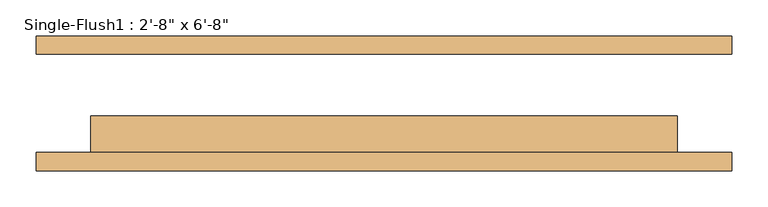
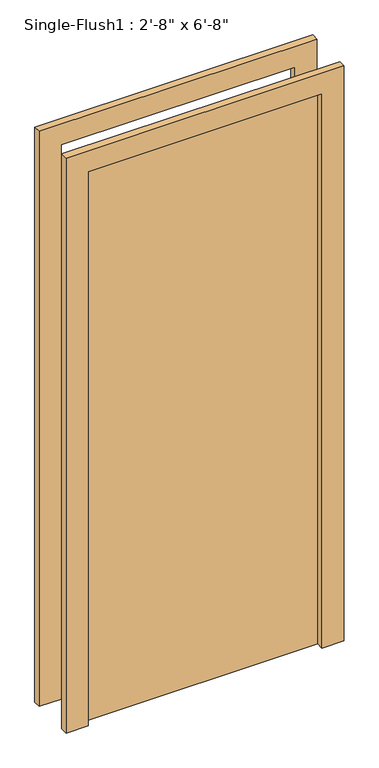
"""IFC4 building model written with IfcOpenShell, lengths in millimetres: door geometry."""

import ifcopenshell
import ifcopenshell.guid

model = None  # the IFC model being written
_history = None  # IfcOwnerHistory: only IFC2X3 demands one
_inside = {}  # id of a spatial element -> (the spatial element, [elements in it])
_under = {}  # id of a project, library or spatial element -> (it, [spatial elements below it])
_declared = {}  # id of a project -> (the project, [libraries it declares])
_typed = {}  # id of a type object -> (the type object, [elements of that type])
_made_of = {}  # id of a material, layer set ... -> (it, [elements and type objects made of it])


def new_model(schema):
    """Start an empty IFC model of exactly this schema.

    Asked for "IFC4X3", IfcOpenShell would pick the latest addendum, in which some entities
    have other attributes; the version numbers below select the first issue.
    IFC2X3 requires an IfcOwnerHistory on every rooted entity: one is made here for all.
    """
    global model, _history
    if schema == "IFC4X3":
        model = ifcopenshell.file(schema_version=(4, 3, 0, 0))
    else:
        model = ifcopenshell.file(schema=schema)
    _inside.clear()
    _under.clear()
    _declared.clear()
    _typed.clear()
    _made_of.clear()
    _history = None
    if model.schema == "IFC2X3":
        org = make("IfcOrganization", Name="unknown")
        user = make(
            "IfcPersonAndOrganization",
            ThePerson=make("IfcPerson", FamilyName="unknown"),
            TheOrganization=org,
        )
        app = make(
            "IfcApplication",
            ApplicationDeveloper=org,
            Version="unknown",
            ApplicationFullName="unknown",
            ApplicationIdentifier="unknown",
        )
        _history = make(
            "IfcOwnerHistory",
            OwningUser=user,
            OwningApplication=app,
            ChangeAction="ADDED",
            CreationDate=0,
        )
    return model


def make(cls, **values):
    """One entity of the class cls with the attributes given. An attribute that is None is left unset."""
    return model.create_entity(
        cls, **{name: value for name, value in values.items() if value is not None}
    )


def rooted(cls, **values):
    """An entity with a GlobalId (a new one), such as an element, a storey or a relation."""
    return make(cls, GlobalId=ifcopenshell.guid.new(), OwnerHistory=_history, **values)


def si_unit(unit_type, name, prefix=None):
    """IfcSIUnit, for example si_unit("LENGTHUNIT", "METRE", prefix="MILLI")."""
    return make("IfcSIUnit", UnitType=unit_type, Prefix=prefix, Name=name)


def assignment(units):
    """IfcUnitAssignment: the units of a project."""
    return None if units is None else make("IfcUnitAssignment", Units=units)


def point(xyz):
    """IfcCartesianPoint."""
    return None if xyz is None else make("IfcCartesianPoint", Coordinates=xyz)


def direction(xyz):
    """IfcDirection."""
    return None if xyz is None else make("IfcDirection", DirectionRatios=xyz)


def frame(location, z_axis=None, x_axis=None):
    """IfcAxis2Placement3D, a coordinate frame: its origin and axes. An axis left out is left unset."""
    return make(
        "IfcAxis2Placement3D",
        Location=point(location),
        Axis=direction(z_axis),
        RefDirection=direction(x_axis),
    )


def origin():
    """The frame at (0, 0, 0) with its axes left unset."""
    return frame((0.0, 0.0, 0.0))


def origin_with_axes():
    """The frame at (0, 0, 0) with the z axis (0, 0, 1) and the x axis (1, 0, 0) written out."""
    return frame((0.0, 0.0, 0.0), z_axis=(0.0, 0.0, 1.0), x_axis=(1.0, 0.0, 0.0))


def place(relative_to, where):
    """IfcLocalPlacement: puts the frame where relative to a parent placement (None: the world)."""
    return make(
        "IfcLocalPlacement", PlacementRelTo=relative_to, RelativePlacement=where
    )


def context(
    kind, dimensions, precision=None, world=None, true_north=None, identifier=None
):
    """IfcGeometricRepresentationContext, for example the 3D "Model" context."""
    return make(
        "IfcGeometricRepresentationContext",
        ContextIdentifier=identifier,
        ContextType=kind,
        CoordinateSpaceDimension=dimensions,
        Precision=precision,
        WorldCoordinateSystem=world,
        TrueNorth=true_north,
    )


def project(units=None, contexts=None):
    """IfcProject with its units and contexts."""
    return rooted(
        "IfcProject",
        Name="project",
        RepresentationContexts=contexts,
        UnitsInContext=assignment(units),
    )


def spatial(cls, under=None, at=None, **own):
    """A site, building, storey or space (cls), placed at a placement, below another one or the project."""
    s = rooted(cls, ObjectPlacement=at, **own)
    if under is not None:
        _under.setdefault(under.id(), (under, []))[1].append(s)
    return s


def polyline(points):
    """IfcPolyline through the points."""
    return make("IfcPolyline", Points=[point(p) for p in points])


def outline(outer, holes=None, kind="AREA"):
    """IfcArbitraryClosedProfileDef: a profile drawn as a closed curve; with holes, ...WithVoids."""
    if holes is None:
        return make("IfcArbitraryClosedProfileDef", ProfileType=kind, OuterCurve=outer)
    return make(
        "IfcArbitraryProfileDefWithVoids",
        ProfileType=kind,
        OuterCurve=outer,
        InnerCurves=holes,
    )


def extrude(swept, where, along, depth):
    """IfcExtrudedAreaSolid: the profile swept, set in the frame where, extruded along a direction by depth."""
    return make(
        "IfcExtrudedAreaSolid",
        SweptArea=swept,
        Position=where,
        ExtrudedDirection=direction(along),
        Depth=depth,
    )


def shape(context_of_items, identifier, shape_type, items):
    """IfcShapeRepresentation: the items that make up one representation, for example the "Body"."""
    return make(
        "IfcShapeRepresentation",
        ContextOfItems=context_of_items,
        RepresentationIdentifier=identifier,
        RepresentationType=shape_type,
        Items=items,
    )


def source(mapping_origin, context_of_items, identifier, shape_type, items):
    """IfcRepresentationMap: a shape defined once, which mapped items show again and again."""
    return make(
        "IfcRepresentationMap",
        MappingOrigin=mapping_origin,
        MappedRepresentation=shape(context_of_items, identifier, shape_type, items),
    )


def transform(
    local_origin,
    x_axis=None,
    y_axis=None,
    z_axis=None,
    scale=None,
    scale2=None,
    scale3=None,
    uniform=True,
):
    """IfcCartesianTransformationOperator3D, or its non-uniform kind. x_axis, y_axis, z_axis: its Axis1, 2, 3."""
    if uniform:
        return make(
            "IfcCartesianTransformationOperator3D",
            Axis1=direction(x_axis),
            Axis2=direction(y_axis),
            LocalOrigin=point(local_origin),
            Scale=scale,
            Axis3=direction(z_axis),
        )
    return make(
        "IfcCartesianTransformationOperator3DnonUniform",
        Axis1=direction(x_axis),
        Axis2=direction(y_axis),
        LocalOrigin=point(local_origin),
        Scale=scale,
        Axis3=direction(z_axis),
        Scale2=scale2,
        Scale3=scale3,
    )


def mapped(mapping_source, mapping_target):
    """IfcMappedItem: shows the shape of a source again, moved by a transform."""
    return make(
        "IfcMappedItem", MappingSource=mapping_source, MappingTarget=mapping_target
    )


def made_of(thing, what):
    """Note that an element or type object is made of a material, layer set ...; save() writes the relation."""
    if what is not None:
        _made_of.setdefault(what.id(), (what, []))[1].append(thing)
    return thing


def element(
    cls,
    number,
    at=None,
    inside=None,
    cuts=None,
    type_object=None,
    material=None,
    context=None,
    identifier="Body",
    shape_type=None,
    held_by="IfcProductDefinitionShape",
    body=None,
    shapes=None,
    **own,
):
    """One element of the class cls, such as IfcWall. Its Tag is "e" and its number.

    at: its placement. inside: the storey or other place that contains it. cuts: it is an
    opening in that element (IfcRelVoidsElement). A single representation is given by context,
    identifier, shape_type and body (its items); several are given by shapes. held_by: the class
    of the entity that holds the representations. save() writes the other relations.
    """
    e = rooted(cls, Tag="e%d" % number, ObjectPlacement=at, **own)
    if body is not None:
        shapes = [shape(context, identifier, shape_type, body)]
    if shapes is not None:
        e.Representation = make(held_by, Representations=shapes)
    if inside is not None:
        _inside.setdefault(inside.id(), (inside, []))[1].append(e)
    if cuts is not None:
        rooted(
            "IfcRelVoidsElement", RelatingBuildingElement=cuts, RelatedOpeningElement=e
        )
    if type_object is not None:
        _typed.setdefault(type_object.id(), (type_object, []))[1].append(e)
    return made_of(e, material)


def aggregate(whole, parts):
    """IfcRelAggregates: a whole, such as a stair, and the parts it consists of."""
    return rooted("IfcRelAggregates", RelatingObject=whole, RelatedObjects=parts)


def save(model, path):
    """Write the relations noted so far, then the file.

    IfcRelAggregates (storeys below a building ...), IfcRelContainedInSpatialStructure (elements
    in a storey), IfcRelDefinesByType, IfcRelAssociatesMaterial and IfcRelDeclares: one each for
    every whole, place, type object, material and project.
    """
    for whole, parts in _under.values():
        aggregate(whole, parts)
    for where, things in _inside.values():
        rooted(
            "IfcRelContainedInSpatialStructure",
            RelatedElements=things,
            RelatingStructure=where,
        )
    for kind, things in _typed.values():
        rooted("IfcRelDefinesByType", RelatedObjects=things, RelatingType=kind)
    for what, things in _made_of.values():
        rooted("IfcRelAssociatesMaterial", RelatedObjects=things, RelatingMaterial=what)
    for by, libraries in _declared.values():
        rooted("IfcRelDeclares", RelatingContext=by, RelatedDefinitions=libraries)
    model.write(path)


def door_a239bf7e(model_context):
    return source(origin(), model_context, "Body", "SweptSolid", [
        extrude(outline(polyline([(2108.2, -482.6), (0.0, -482.6), (0.0, -406.4), (2032.0, -406.4), (2032.0, 406.4), (0.0, 406.4), (0.0, 482.6), (2108.2, 482.6), (2108.2, -482.6)])), frame((0.0, -93.6625, 0.0), z_axis=(0.0, 1.0, 0.0), x_axis=(0.0, 0.0, 1.0)), (0.0, 0.0, 1.0), 25.4),
        extrude(outline(polyline([(2108.2, 482.6), (2108.2, -482.6), (0.0, -482.6), (0.0, -406.4), (2032.0, -406.4), (2032.0, 406.4), (0.0, 406.4), (0.0, 482.6), (2108.2, 482.6)])), frame((0.0, 68.2625, 0.0), z_axis=(0.0, 1.0, 0.0), x_axis=(0.0, 0.0, 1.0)), (0.0, 0.0, 1.0), 25.4),
        extrude(outline(polyline([(406.4, -17.4625), (406.4, -68.2625), (-406.4, -68.2625), (-406.4, -17.4625), (406.4, -17.4625)])), origin_with_axes(), (0.0, 0.0, 1.0), 2032.0),
    ])


if __name__ == "__main__":
    model = new_model("IFC4")
    model_context = context("Model", 3, world=origin())
    ifc_project = project(units=[si_unit("LENGTHUNIT", "METRE", prefix="MILLI")], contexts=[model_context])
    site = spatial("IfcSite", under=ifc_project)
    building = spatial("IfcBuilding", under=site)
    placement = place(None, origin())
    door_shape = door_a239bf7e(model_context)
    element("IfcDoor", 1, ObjectType="Single-Flush1 : 2'-8\" x 6'-8\"", at=placement, inside=building, context=model_context, shape_type="MappedRepresentation", body=[
        mapped(door_shape, transform((0.0, 0.0, 0.0), x_axis=(1.0, 0.0, 0.0), y_axis=(0.0, 1.0, 0.0), z_axis=(0.0, 0.0, 1.0))),
    ])
    save(model, "model.ifc")

# Revit data of these elements
# Type "Single-Flush1 : 2'-8\" x 6'-8\""
#   Type Mark = "23"
#   Construction Type Id = "MDOOR"
#   Assembly Code = "C1020"
#   Analytic Construction = "Metal"
#   Thickness = 0' - 2"
#   Heat Transfer Coefficient (U) = 3.7021 W/(m²·K)
#   Height = 6' - 8"
#   Trim Projection Ext = 0' - 1"
#   Trim Projection Int = 0' - 1"
#   Trim Width = 0' - 3"
#   Width = 2' - 8"
#   Door Material = Door - Panel
#   Frame Material = Door - Frame
#   Visual Light Transmittance = 0
#   Solar Heat Gain Coefficient = 0
#   Function = (empty or 0)
#   Wall Closure = (empty or 0)
# Element 1 (IfcDoor, "Single-Flush1 : 2'-8\" x 6'-8\"")
#   Materials on its faces: "Door - Frame", "Door - Panel"
# Materials
#   "Door - Panel": class "Wood", colour RGB 210 159 95, transparency 0, Cost = 0
#   "Door - Frame": class "Miscellaneous", colour RGB 118 70 51, transparency 0, Cost = 0
